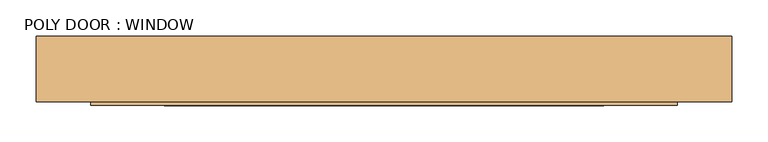
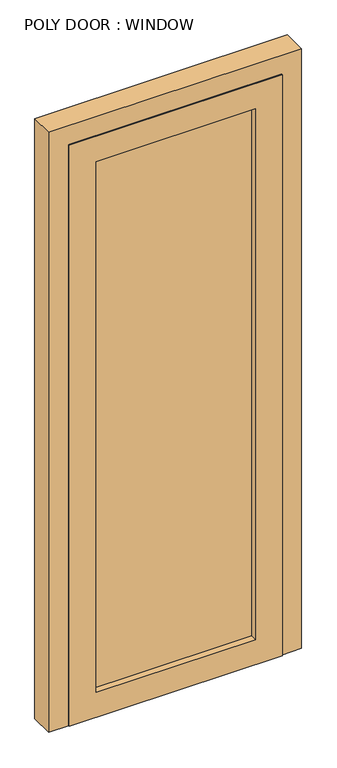
"""IFC4 building model written with IfcOpenShell, lengths in millimetres: door geometry, POLY DOOR : WINDOW."""

from ifc_helpers import new_model, si_unit, frame, origin, place, context, project, spatial, polyline, outline, extrude, source, transform, mapped, element, save


def poly_door_window_e564bd3f(model_context):
    return source(origin(), model_context, "Body", "SweptSolid", [
        extrude(outline(polyline([(304.8, -25.4), (-304.8, -25.4), (-304.8, -12.7), (304.8, -12.7), (304.8, -25.4)])), frame((0.0, 0.0, 101.6), z_axis=(0.0, 0.0, 1.0), x_axis=(1.0, 0.0, 0.0)), (0.0, 0.0, 1.0), 2139.95),
        extrude(outline(polyline([(2343.15, 406.4), (2343.15, -406.4), (0.0, -406.4), (0.0, 406.4), (2343.15, 406.4)]), holes=[polyline([(2241.55, 304.8), (101.6, 304.8), (101.6, -304.8), (2241.55, -304.8), (2241.55, 304.8)])]), frame((0.0, -50.8, 0.0), z_axis=(0.0, 1.0, 0.0), x_axis=(0.0, 0.0, 1.0)), (0.0, 0.0, 1.0), 50.8),
        extrude(outline(polyline([(2419.35, -482.6), (0.0, -482.6), (0.0, -406.4), (2343.15, -406.4), (2343.15, 406.4), (0.0, 406.4), (0.0, 482.6), (2419.35, 482.6), (2419.35, -482.6)])), frame((0.0, -45.39996, 0.0), z_axis=(0.0, 1.0, 0.0), x_axis=(0.0, 0.0, 1.0)), (0.0, 0.0, 1.0), 90.79992),
    ])


if __name__ == "__main__":
    model = new_model("IFC4")
    model_context = context("Model", 3, world=origin())
    ifc_project = project(units=[si_unit("LENGTHUNIT", "METRE", prefix="MILLI")], contexts=[model_context])
    site = spatial("IfcSite", under=ifc_project)
    building = spatial("IfcBuilding", under=site)
    placement = place(None, origin())
    poly_door_window_shape = poly_door_window_e564bd3f(model_context)
    element("IfcDoor", 1, ObjectType="POLY DOOR : WINDOW", at=placement, inside=building, context=model_context, shape_type="MappedRepresentation", body=[
        mapped(poly_door_window_shape, transform((0.0, 0.0, 0.0), x_axis=(1.0, 0.0, 0.0), y_axis=(0.0, 1.0, 0.0), z_axis=(0.0, 0.0, 1.0))),
    ])
    save(model, "model.ifc")

# Revit data of these elements
# Type "POLY DOOR : WINDOW"
#   Type Mark = "58"
#   Assembly Code = "C1020"
#   Analytic Construction = "<None>"
#   Thickness = 0' - 2"
#   Glass Inset = 0' - 4"
#   Height = 7' - 8 1/4"
#   Trim Projection Ext = 0' - 1"
#   Trim Projection Int = 0' - 1"
#   Trim Width = 0' - 3"
#   Width = 2' - 8"
#   WINDOW = no
#   Glass Material = ALUM. STOREFRONT W/ INSULATED GLAZING
#   Door Material = Aluminum
#   Frame Material = Aluminum
#   Function = (empty or 0)
#   Wall Closure = (empty or 0)
# Element 1 (IfcDoor, "POLY DOOR : WINDOW")
#   Materials on its faces: "Aluminum", "ALUM. STOREFRONT W/ INSULATED GLAZING"
# Materials
#   "ALUM. STOREFRONT W/ INSULATED GLAZING": class "Glass", colour RGB 196 205 210, transparency 0.85, Description = "Soda Lime Glass", Cost = 0
#   "Aluminum": class "Metal", colour RGB 244 244 244, transparency 0, Description = "Aluminum 6061", Cost = 0
